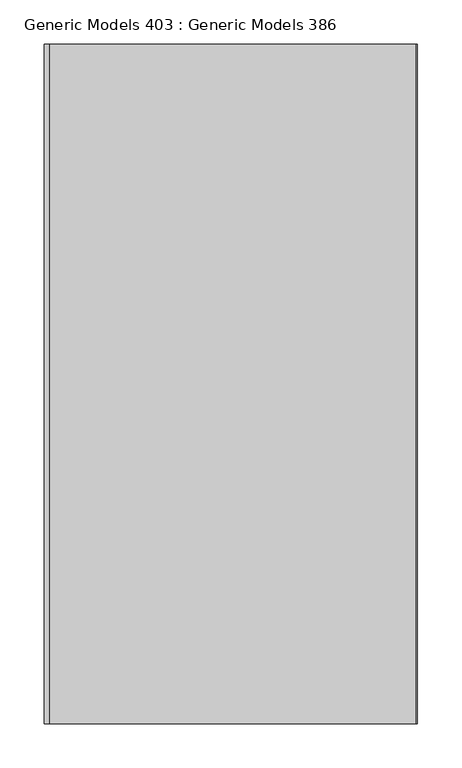
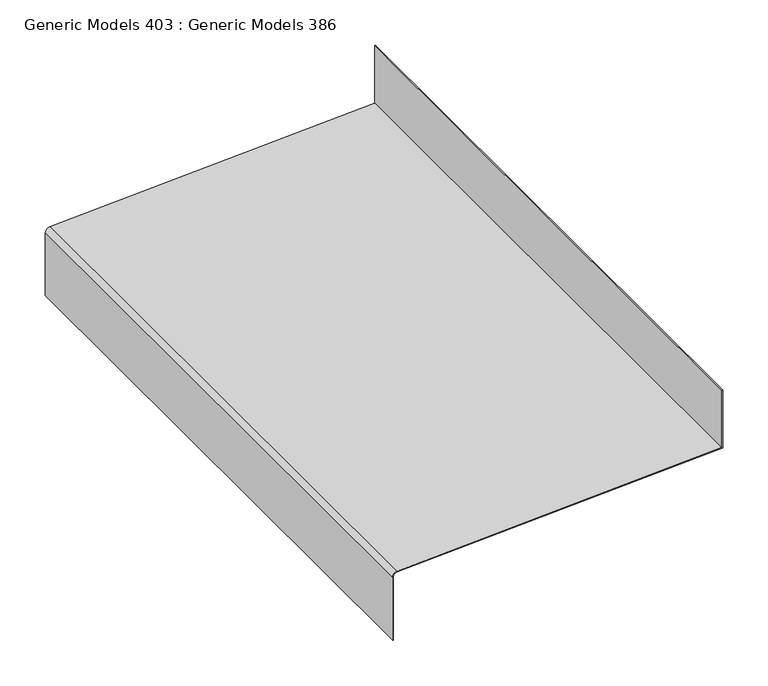
"""IFC4 building model written with IfcOpenShell, lengths in millimetres: proxy geometry, Generic Models 403 : Generic Models 386."""

from ifc_helpers import new_model, si_unit, point, frame, frame_2d, origin, place, context, project, spatial, polyline, circle_curve, trimmed, segment, composite_curve, outline, extrude, source, transform, mapped, element, save


def generic_models_403_generic_models_386_3df1fb79(model_context):
    return source(origin(), model_context, "Body", "SweptSolid", [
        extrude(outline(composite_curve([segment(polyline([(129137.9419919, -6631.9548796), (129116.330443, -7044.3277971)]), True, "CONTINUOUS"), segment(trimmed(circle_curve(frame_2d((129109.9891455, -7043.9954637)), 6.35), [point((129116.330443, -7044.3277971))], [point((129109.9891455, -7050.3454637))], False, "CARTESIAN"), True, "CONTINUOUS"), segment(polyline([(129109.9891455, -7050.3454637), (129025.396, -7050.3454637), (129025.396, -7049.5517137), (129109.9891455, -7049.5517137)]), True, "CONTINUOUS"), segment(trimmed(circle_curve(frame_2d((129109.9891455, -7043.9954637)), 5.55625), [point((129109.9891455, -7049.5517137))], [point((129115.5377808, -7044.2862554))], True, "CARTESIAN"), True, "CONTINUOUS"), segment(polyline([(129115.5377808, -7044.2862554), (129137.1887513, -6631.1611296), (129215.0570554, -6631.1611296), (129215.0570554, -6631.9548796), (129137.9419919, -6631.9548796)]), True, "CONTINUOUS")], self_intersect=False)), frame((0.0, -4250.542257, 0.0), z_axis=(0.0, 1.0, 0.0), x_axis=(0.0, 0.0, 1.0)), (0.0, 0.0, 1.0), 763.8192232),
    ])


if __name__ == "__main__":
    model = new_model("IFC4")
    model_context = context("Model", 3, world=origin())
    ifc_project = project(units=[si_unit("LENGTHUNIT", "METRE", prefix="MILLI")], contexts=[model_context])
    site = spatial("IfcSite", under=ifc_project)
    building = spatial("IfcBuilding", under=site)
    placement = place(None, origin())
    generic_models_403_generic_models_386_shape = generic_models_403_generic_models_386_3df1fb79(model_context)
    element("IfcBuildingElementProxy", 1, Name="Generic Models 403 : Generic Models 386", ObjectType="Generic Models 403 : Generic Models 386", at=placement, inside=building, context=model_context, shape_type="MappedRepresentation", body=[
        mapped(generic_models_403_generic_models_386_shape, transform((0.0, 0.0, 0.0), x_axis=(1.0, 0.0, 0.0), y_axis=(0.0, 1.0, 0.0), z_axis=(0.0, 0.0, 1.0))),
    ])
    save(model, "model.ifc")

# Revit data of these elements
# Element 1 (IfcBuildingElementProxy, "Generic Models 403 : Generic Models 386")
#   Materials on its faces: "_(2) LAYERS NO. 30 ASTM D226 ASPHALT SATURATED ORGANIC FELT @ ROOF"
# Materials
#   "_(2) LAYERS NO. 30 ASTM D226 ASPHALT SATURATED ORGANIC FELT @ ROOF": class "Generic", colour RGB 67 154 161, transparency 0, Cost = 0
